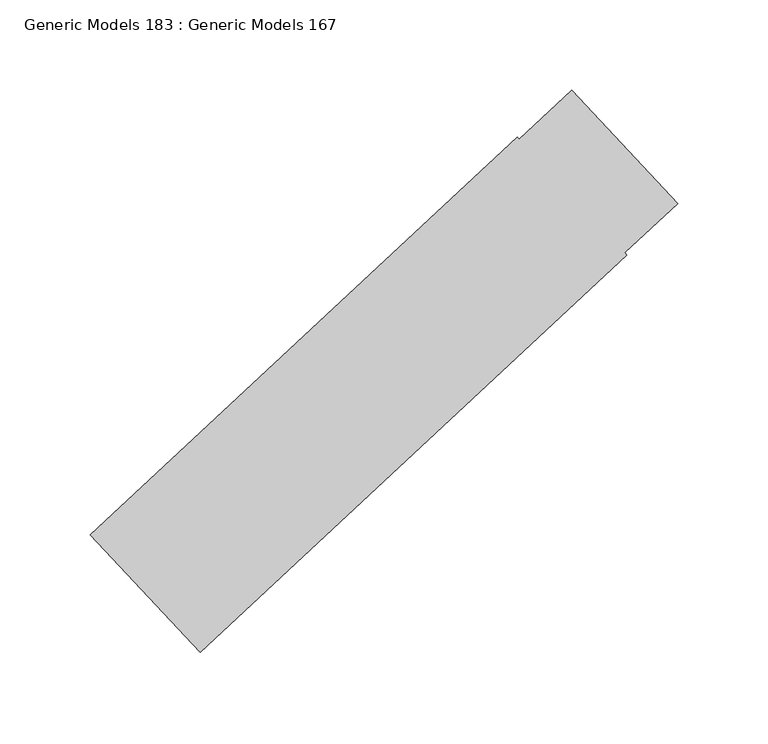
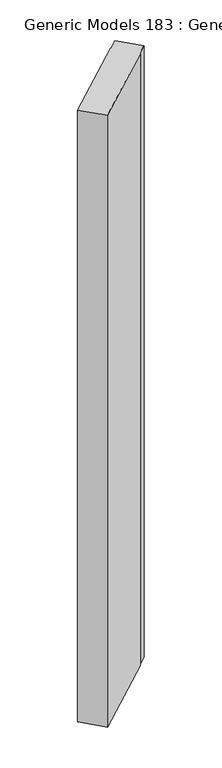
"""IFC4 building model written with IfcOpenShell, lengths in millimetres: proxy geometry, Generic Models 183 : Generic Models 167."""

import ifcopenshell
import ifcopenshell.guid

model = None  # the IFC model being written
_history = None  # IfcOwnerHistory: only IFC2X3 demands one
_inside = {}  # id of a spatial element -> (the spatial element, [elements in it])
_under = {}  # id of a project, library or spatial element -> (it, [spatial elements below it])
_declared = {}  # id of a project -> (the project, [libraries it declares])
_typed = {}  # id of a type object -> (the type object, [elements of that type])
_made_of = {}  # id of a material, layer set ... -> (it, [elements and type objects made of it])


def new_model(schema):
    """Start an empty IFC model of exactly this schema.

    Asked for "IFC4X3", IfcOpenShell would pick the latest addendum, in which some entities
    have other attributes; the version numbers below select the first issue.
    IFC2X3 requires an IfcOwnerHistory on every rooted entity: one is made here for all.
    """
    global model, _history
    if schema == "IFC4X3":
        model = ifcopenshell.file(schema_version=(4, 3, 0, 0))
    else:
        model = ifcopenshell.file(schema=schema)
    _inside.clear()
    _under.clear()
    _declared.clear()
    _typed.clear()
    _made_of.clear()
    _history = None
    if model.schema == "IFC2X3":
        org = make("IfcOrganization", Name="unknown")
        user = make(
            "IfcPersonAndOrganization",
            ThePerson=make("IfcPerson", FamilyName="unknown"),
            TheOrganization=org,
        )
        app = make(
            "IfcApplication",
            ApplicationDeveloper=org,
            Version="unknown",
            ApplicationFullName="unknown",
            ApplicationIdentifier="unknown",
        )
        _history = make(
            "IfcOwnerHistory",
            OwningUser=user,
            OwningApplication=app,
            ChangeAction="ADDED",
            CreationDate=0,
        )
    return model


def make(cls, **values):
    """One entity of the class cls with the attributes given. An attribute that is None is left unset."""
    return model.create_entity(
        cls, **{name: value for name, value in values.items() if value is not None}
    )


def rooted(cls, **values):
    """An entity with a GlobalId (a new one), such as an element, a storey or a relation."""
    return make(cls, GlobalId=ifcopenshell.guid.new(), OwnerHistory=_history, **values)


def si_unit(unit_type, name, prefix=None):
    """IfcSIUnit, for example si_unit("LENGTHUNIT", "METRE", prefix="MILLI")."""
    return make("IfcSIUnit", UnitType=unit_type, Prefix=prefix, Name=name)


def assignment(units):
    """IfcUnitAssignment: the units of a project."""
    return None if units is None else make("IfcUnitAssignment", Units=units)


def point(xyz):
    """IfcCartesianPoint."""
    return None if xyz is None else make("IfcCartesianPoint", Coordinates=xyz)


def direction(xyz):
    """IfcDirection."""
    return None if xyz is None else make("IfcDirection", DirectionRatios=xyz)


def frame(location, z_axis=None, x_axis=None):
    """IfcAxis2Placement3D, a coordinate frame: its origin and axes. An axis left out is left unset."""
    return make(
        "IfcAxis2Placement3D",
        Location=point(location),
        Axis=direction(z_axis),
        RefDirection=direction(x_axis),
    )


def origin():
    """The frame at (0, 0, 0) with its axes left unset."""
    return frame((0.0, 0.0, 0.0))


def origin_with_axes():
    """The frame at (0, 0, 0) with the z axis (0, 0, 1) and the x axis (1, 0, 0) written out."""
    return frame((0.0, 0.0, 0.0), z_axis=(0.0, 0.0, 1.0), x_axis=(1.0, 0.0, 0.0))


def place(relative_to, where):
    """IfcLocalPlacement: puts the frame where relative to a parent placement (None: the world)."""
    return make(
        "IfcLocalPlacement", PlacementRelTo=relative_to, RelativePlacement=where
    )


def context(
    kind, dimensions, precision=None, world=None, true_north=None, identifier=None
):
    """IfcGeometricRepresentationContext, for example the 3D "Model" context."""
    return make(
        "IfcGeometricRepresentationContext",
        ContextIdentifier=identifier,
        ContextType=kind,
        CoordinateSpaceDimension=dimensions,
        Precision=precision,
        WorldCoordinateSystem=world,
        TrueNorth=true_north,
    )


def project(units=None, contexts=None):
    """IfcProject with its units and contexts."""
    return rooted(
        "IfcProject",
        Name="project",
        RepresentationContexts=contexts,
        UnitsInContext=assignment(units),
    )


def spatial(cls, under=None, at=None, **own):
    """A site, building, storey or space (cls), placed at a placement, below another one or the project."""
    s = rooted(cls, ObjectPlacement=at, **own)
    if under is not None:
        _under.setdefault(under.id(), (under, []))[1].append(s)
    return s


def polyline(points):
    """IfcPolyline through the points."""
    return make("IfcPolyline", Points=[point(p) for p in points])


def outline(outer, holes=None, kind="AREA"):
    """IfcArbitraryClosedProfileDef: a profile drawn as a closed curve; with holes, ...WithVoids."""
    if holes is None:
        return make("IfcArbitraryClosedProfileDef", ProfileType=kind, OuterCurve=outer)
    return make(
        "IfcArbitraryProfileDefWithVoids",
        ProfileType=kind,
        OuterCurve=outer,
        InnerCurves=holes,
    )


def extrude(swept, where, along, depth):
    """IfcExtrudedAreaSolid: the profile swept, set in the frame where, extruded along a direction by depth."""
    return make(
        "IfcExtrudedAreaSolid",
        SweptArea=swept,
        Position=where,
        ExtrudedDirection=direction(along),
        Depth=depth,
    )


def shape(context_of_items, identifier, shape_type, items):
    """IfcShapeRepresentation: the items that make up one representation, for example the "Body"."""
    return make(
        "IfcShapeRepresentation",
        ContextOfItems=context_of_items,
        RepresentationIdentifier=identifier,
        RepresentationType=shape_type,
        Items=items,
    )


def source(mapping_origin, context_of_items, identifier, shape_type, items):
    """IfcRepresentationMap: a shape defined once, which mapped items show again and again."""
    return make(
        "IfcRepresentationMap",
        MappingOrigin=mapping_origin,
        MappedRepresentation=shape(context_of_items, identifier, shape_type, items),
    )


def transform(
    local_origin,
    x_axis=None,
    y_axis=None,
    z_axis=None,
    scale=None,
    scale2=None,
    scale3=None,
    uniform=True,
):
    """IfcCartesianTransformationOperator3D, or its non-uniform kind. x_axis, y_axis, z_axis: its Axis1, 2, 3."""
    if uniform:
        return make(
            "IfcCartesianTransformationOperator3D",
            Axis1=direction(x_axis),
            Axis2=direction(y_axis),
            LocalOrigin=point(local_origin),
            Scale=scale,
            Axis3=direction(z_axis),
        )
    return make(
        "IfcCartesianTransformationOperator3DnonUniform",
        Axis1=direction(x_axis),
        Axis2=direction(y_axis),
        LocalOrigin=point(local_origin),
        Scale=scale,
        Axis3=direction(z_axis),
        Scale2=scale2,
        Scale3=scale3,
    )


def mapped(mapping_source, mapping_target):
    """IfcMappedItem: shows the shape of a source again, moved by a transform."""
    return make(
        "IfcMappedItem", MappingSource=mapping_source, MappingTarget=mapping_target
    )


def made_of(thing, what):
    """Note that an element or type object is made of a material, layer set ...; save() writes the relation."""
    if what is not None:
        _made_of.setdefault(what.id(), (what, []))[1].append(thing)
    return thing


def element(
    cls,
    number,
    at=None,
    inside=None,
    cuts=None,
    type_object=None,
    material=None,
    context=None,
    identifier="Body",
    shape_type=None,
    held_by="IfcProductDefinitionShape",
    body=None,
    shapes=None,
    **own,
):
    """One element of the class cls, such as IfcWall. Its Tag is "e" and its number.

    at: its placement. inside: the storey or other place that contains it. cuts: it is an
    opening in that element (IfcRelVoidsElement). A single representation is given by context,
    identifier, shape_type and body (its items); several are given by shapes. held_by: the class
    of the entity that holds the representations. save() writes the other relations.
    """
    e = rooted(cls, Tag="e%d" % number, ObjectPlacement=at, **own)
    if body is not None:
        shapes = [shape(context, identifier, shape_type, body)]
    if shapes is not None:
        e.Representation = make(held_by, Representations=shapes)
    if inside is not None:
        _inside.setdefault(inside.id(), (inside, []))[1].append(e)
    if cuts is not None:
        rooted(
            "IfcRelVoidsElement", RelatingBuildingElement=cuts, RelatedOpeningElement=e
        )
    if type_object is not None:
        _typed.setdefault(type_object.id(), (type_object, []))[1].append(e)
    return made_of(e, material)


def aggregate(whole, parts):
    """IfcRelAggregates: a whole, such as a stair, and the parts it consists of."""
    return rooted("IfcRelAggregates", RelatingObject=whole, RelatedObjects=parts)


def save(model, path):
    """Write the relations noted so far, then the file.

    IfcRelAggregates (storeys below a building ...), IfcRelContainedInSpatialStructure (elements
    in a storey), IfcRelDefinesByType, IfcRelAssociatesMaterial and IfcRelDeclares: one each for
    every whole, place, type object, material and project.
    """
    for whole, parts in _under.values():
        aggregate(whole, parts)
    for where, things in _inside.values():
        rooted(
            "IfcRelContainedInSpatialStructure",
            RelatedElements=things,
            RelatingStructure=where,
        )
    for kind, things in _typed.values():
        rooted("IfcRelDefinesByType", RelatedObjects=things, RelatingType=kind)
    for what, things in _made_of.values():
        rooted("IfcRelAssociatesMaterial", RelatedObjects=things, RelatingMaterial=what)
    for by, libraries in _declared.values():
        rooted("IfcRelDeclares", RelatingContext=by, RelatedDefinitions=libraries)
    model.write(path)


def generic_models_183_generic_models_167_0fd02149(model_context):
    return source(origin(), model_context, "Body", "SweptSolid", [
        extrude(outline(polyline([(58274.9742538, 3399.4755786), (58510.7156694, 3619.3080052), (58511.7983418, 3618.1469812), (58540.8239419, 3645.2137911), (58599.2882513, 3582.518495), (58570.2626513, 3555.4516851), (58571.3453237, 3554.2906611), (58335.603908, 3334.4582346), (58274.9742538, 3399.4755786)])), origin_with_axes(), (0.0, 0.0, 1.0), 2133.6),
    ])


if __name__ == "__main__":
    model = new_model("IFC4")
    model_context = context("Model", 3, world=origin())
    ifc_project = project(units=[si_unit("LENGTHUNIT", "METRE", prefix="MILLI")], contexts=[model_context])
    site = spatial("IfcSite", under=ifc_project)
    building = spatial("IfcBuilding", under=site)
    placement = place(None, origin())
    generic_models_183_generic_models_167_shape = generic_models_183_generic_models_167_0fd02149(model_context)
    element("IfcBuildingElementProxy", 1, Name="Generic Models 183 : Generic Models 167", ObjectType="Generic Models 183 : Generic Models 167", at=placement, inside=building, context=model_context, shape_type="MappedRepresentation", body=[
        mapped(generic_models_183_generic_models_167_shape, transform((0.0, 0.0, 0.0), x_axis=(1.0, 0.0, 0.0), y_axis=(0.0, 1.0, 0.0), z_axis=(0.0, 0.0, 1.0))),
    ])
    save(model, "model.ifc")

# Revit data of these elements
# Element 1 (IfcBuildingElementProxy, "Generic Models 183 : Generic Models 167")
#   Materials on its faces: "METAL STUDS (MATCH EXISTING SIZE/GAUGE/SPACING)"
# Materials
#   "METAL STUDS (MATCH EXISTING SIZE/GAUGE/SPACING)": class "Unassigned", colour RGB 210 209 208, transparency 0, Keynote = "M05121300.02", Cost = 0
